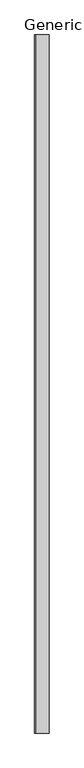
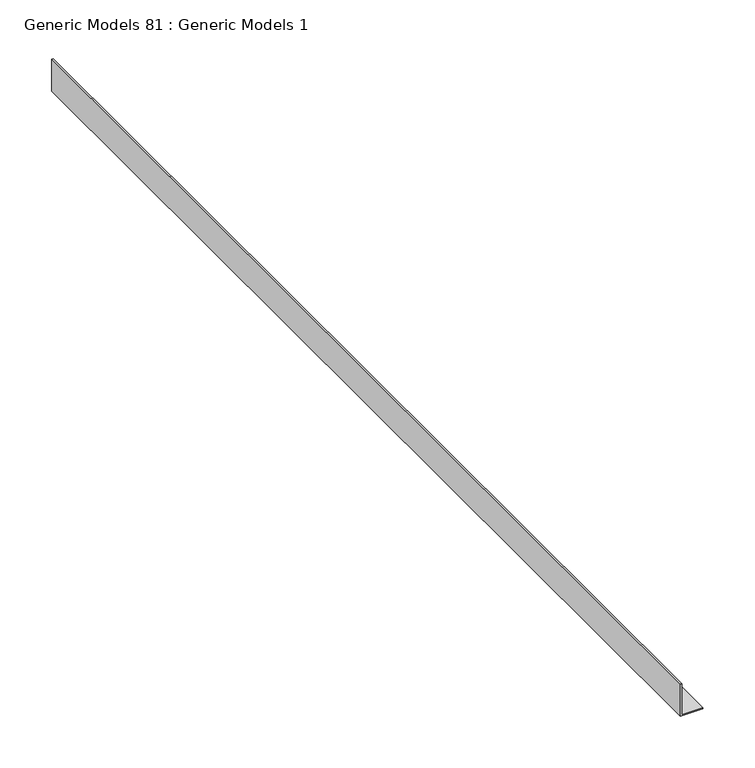
"""IFC4 building model written with IfcOpenShell, lengths in millimetres: proxy geometry, Generic Models 81 : Generic Models 1."""

from ifc_helpers import new_model, si_unit, frame, origin, place, context, project, spatial, polyline, outline, extrude, source, transform, mapped, element, save


def generic_models_81_generic_models_1_62cb9d11(model_context):
    return source(origin(), model_context, "Body", "SweptSolid", [
        extrude(outline(polyline([(2304.9709098, 49799.875), (2266.8709098, 49799.875), (2266.8709098, 49825.275), (2268.4584098, 49825.275), (2268.4584098, 49801.4625), (2304.9709098, 49801.4625), (2304.9709098, 49799.875)])), frame((0.0, 0.0, 0.0), z_axis=(0.0, 1.0, 0.0), x_axis=(0.0, 0.0, 1.0)), (0.0, 0.0, 1.0), 1219.2),
    ])


if __name__ == "__main__":
    model = new_model("IFC4")
    model_context = context("Model", 3, world=origin())
    ifc_project = project(units=[si_unit("LENGTHUNIT", "METRE", prefix="MILLI")], contexts=[model_context])
    site = spatial("IfcSite", under=ifc_project)
    building = spatial("IfcBuilding", under=site)
    placement = place(None, origin())
    generic_models_81_generic_models_1_shape = generic_models_81_generic_models_1_62cb9d11(model_context)
    element("IfcBuildingElementProxy", 1, Name="Generic Models 81 : Generic Models 1", ObjectType="Generic Models 81 : Generic Models 1", at=placement, inside=building, context=model_context, shape_type="MappedRepresentation", body=[
        mapped(generic_models_81_generic_models_1_shape, transform((0.0, 0.0, 0.0), x_axis=(1.0, 0.0, 0.0), y_axis=(0.0, 1.0, 0.0), z_axis=(0.0, 0.0, 1.0))),
    ])
    save(model, "model.ifc")

# Revit data of these elements
# Element 1 (IfcBuildingElementProxy, "Generic Models 81 : Generic Models 1")
#   Materials on its faces: "CEILING TRACK AS SCHEDULED"
# Materials
#   "CEILING TRACK AS SCHEDULED": class "Unassigned", colour RGB 210 209 208, transparency 0, Keynote = "M05121300.02", Cost = 0
